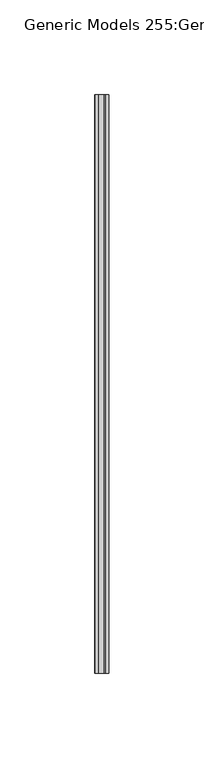
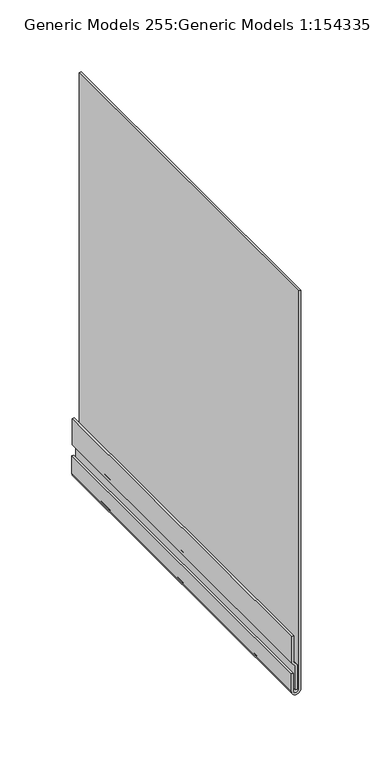
"""IFC4 building model written with IfcOpenShell, lengths in millimetres: proxy geometry, Generic Models 255:Generic Models 1:154335 : Generic Models 255:Generic Models 1:154335."""

from ifc_helpers import new_model, si_unit, point, frame, frame_2d, origin, place, context, project, spatial, polyline, circle_curve, trimmed, segment, composite_curve, outline, extrude, source, transform, mapped, element, save


def generic_models_255_generic_models_1_154335_generic_models_911f2678(model_context):
    return source(origin(), model_context, "Body", "SweptSolid", [
        extrude(outline(polyline([(6038.7355217, 2083.8444695), (6059.5390463, 2083.8444695), (6062.9983174, 2081.090713), (6084.8963279, 2081.090713), (6084.8963279, 2079.503213), (6062.4436021, 2079.503213), (6058.984331, 2082.2569695), (6038.7355217, 2082.2569695), (6038.7355217, 2083.8444695)])), frame((0.0, 5312.3878092, 0.0), z_axis=(0.0, 1.0, 0.0), x_axis=(0.0, 0.0, 1.0)), (0.0, 0.0, 1.0), 304.8),
        extrude(outline(composite_curve([segment(polyline([(6053.4881548, 2079.2507374), (6038.2359325, 2079.2507374)]), True, "CONTINUOUS"), segment(trimmed(circle_curve(frame_2d((6038.2359325, 2082.9244946)), 3.6737572), [point((6038.2359325, 2079.2507374))], [point((6038.2359325, 2086.5982518))], False, "CARTESIAN"), True, "CONTINUOUS"), segment(polyline([(6038.2359325, 2086.5982518), (6376.1796366, 2086.5982518), (6376.1796366, 2085.0107518), (6038.2359325, 2085.0107518)]), True, "CONTINUOUS"), segment(trimmed(circle_curve(frame_2d((6038.2359325, 2082.9244946)), 2.0862572), [point((6038.2359325, 2085.0107518))], [point((6038.2359325, 2080.8382374))], True, "CARTESIAN"), True, "CONTINUOUS"), segment(polyline([(6038.2359325, 2080.8382374), (6053.4881548, 2080.8382374), (6053.4881548, 2079.2507374)]), True, "CONTINUOUS")], self_intersect=False)), frame((0.0, 5312.3878092, 0.0), z_axis=(0.0, 1.0, 0.0), x_axis=(0.0, 0.0, 1.0)), (0.0, 0.0, 1.0), 304.8),
    ])


if __name__ == "__main__":
    model = new_model("IFC4")
    model_context = context("Model", 3, world=origin())
    ifc_project = project(units=[si_unit("LENGTHUNIT", "METRE", prefix="MILLI")], contexts=[model_context])
    site = spatial("IfcSite", under=ifc_project)
    building = spatial("IfcBuilding", under=site)
    placement = place(None, origin())
    generic_models_255_generic_models_1_154335_generic_models_shape = generic_models_255_generic_models_1_154335_generic_models_911f2678(model_context)
    element("IfcBuildingElementProxy", 1, Name="Generic Models 255:Generic Models 1:154335 : Generic Models 255:Generic Models 1:154335", ObjectType="Generic Models 255:Generic Models 1:154335 : Generic Models 255:Generic Models 1:154335", at=placement, inside=building, context=model_context, shape_type="MappedRepresentation", body=[
        mapped(generic_models_255_generic_models_1_154335_generic_models_shape, transform((0.0, 0.0, 0.0), x_axis=(1.0, 0.0, 0.0), y_axis=(0.0, 1.0, 0.0), z_axis=(0.0, 0.0, 1.0))),
    ])
    save(model, "model.ifc")

# Revit data of these elements
# Type "Generic Models 255:Generic Models 1:154335 : Generic Models 255:Generic Models 1:154335"
#   NameOverride = "Generic Models 255:Generic Models 1:154335"
#   ObjectTypeOverride = "Generic Models 255:Generic Models 1"
#   Reference = "Generic Models 1"
#   Category = "Generic Models"
#   Tag = "154335"
# Element 1 (IfcBuildingElementProxy, "Generic Models 255:Generic Models 1:154335 : Generic Models 255:Generic Models 1:154335")
#   Materials on its faces: "_16 GA. COPPER BRAKE METAL FASCIA 21960"
# Materials
#   "_16 GA. COPPER BRAKE METAL FASCIA 21960": class "Unassigned", colour RGB 175 175 175, transparency 0
